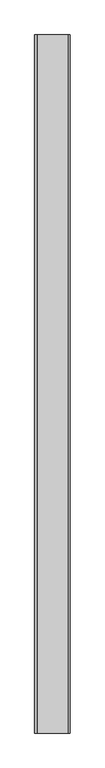
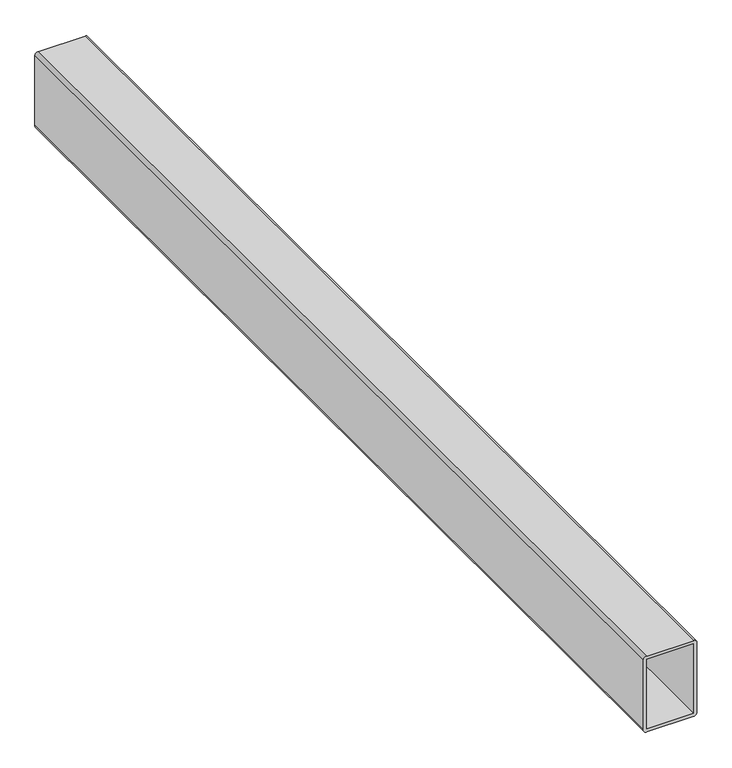
"""IFC4 building model written with IfcOpenShell, lengths in millimetres: proxy geometry, Door frame001 11519 : Door frame001 11519."""

from ifc_helpers import new_model, si_unit, point, frame, frame_2d, origin, place, context, project, spatial, polyline, circle_curve, trimmed, segment, composite_curve, outline, extrude, source, transform, mapped, element, save


def generic_models_2a17c90b(model_context):
    return source(origin(), model_context, "Body", "SweptSolid", [
        extrude(outline(composite_curve([segment(polyline([(32616.0375625, -8390.3106967), (32616.0375625, -8301.4106967)]), True, "CONTINUOUS"), segment(trimmed(circle_curve(frame_2d((32622.3875625, -8301.4106967)), 6.35), [point((32616.0375625, -8301.4106967))], [point((32622.3875625, -8295.0606967))], False, "CARTESIAN"), True, "CONTINUOUS"), segment(polyline([(32622.3875625, -8295.0606967), (32762.0875625, -8295.0606967)]), True, "CONTINUOUS"), segment(trimmed(circle_curve(frame_2d((32762.0875625, -8301.4106967)), 6.35), [point((32762.0875625, -8295.0606967))], [point((32768.4375625, -8301.4106967))], False, "CARTESIAN"), True, "CONTINUOUS"), segment(polyline([(32768.4375625, -8301.4106967), (32768.4375625, -8390.3106967)]), True, "CONTINUOUS"), segment(trimmed(circle_curve(frame_2d((32762.0875625, -8390.3106967)), 6.35), [point((32768.4375625, -8390.3106967))], [point((32762.0875625, -8396.6606967))], False, "CARTESIAN"), True, "CONTINUOUS"), segment(polyline([(32762.0875625, -8396.6606967), (32622.3875625, -8396.6606967)]), True, "CONTINUOUS"), segment(trimmed(circle_curve(frame_2d((32622.3875625, -8390.3106967)), 6.35), [point((32622.3875625, -8396.6606967))], [point((32616.0375625, -8390.3106967))], False, "CARTESIAN"), True, "CONTINUOUS")], self_intersect=False), holes=[polyline([(32761.9375625, -8301.5606967), (32622.5375625, -8301.5606967), (32622.5375625, -8390.1606967), (32761.9375625, -8390.1606967), (32761.9375625, -8301.5606967)])]), frame((0.0, 4540.4513244, 0.0), z_axis=(0.0, 1.0, 0.0), x_axis=(0.0, 0.0, 1.0)), (0.0, 0.0, 1.0), 2000.0),
    ])


if __name__ == "__main__":
    model = new_model("IFC4")
    model_context = context("Model", 3, world=origin())
    ifc_project = project(units=[si_unit("LENGTHUNIT", "METRE", prefix="MILLI")], contexts=[model_context])
    site = spatial("IfcSite", under=ifc_project)
    building = spatial("IfcBuilding", under=site)
    placement = place(None, origin())
    generic_models_shape = generic_models_2a17c90b(model_context)
    element("IfcBuildingElementProxy", 1, Name="Door frame001 11519 : Door frame001 11519", ObjectType="Door frame001 11519 : Door frame001 11519", at=placement, inside=building, context=model_context, shape_type="MappedRepresentation", body=[
        mapped(generic_models_shape, transform((0.0, 0.0, 0.0), x_axis=(1.0, 0.0, 0.0), y_axis=(0.0, 1.0, 0.0), z_axis=(0.0, 0.0, 1.0))),
    ])
    save(model, "model.ifc")

# Revit data of these elements
# Type "Door frame001 11519 : Door frame001 11519"
#   NameOverride = "Door frame001"
# Element 1 (IfcBuildingElementProxy, "Door frame001 11519 : Door frame001 11519")
#   Materials on its faces: "DOOR FRAME: TUBE STEEL PROFILE - METALIZED, PRIMED & PAINTED (COLOR PER ARCHITECT)"
# Materials
#   "DOOR FRAME: TUBE STEEL PROFILE - METALIZED, PRIMED & PAINTED (COLOR PER ARCHITECT)": class "Unassigned", colour RGB 128 128 128, transparency 0, Cost = 0
